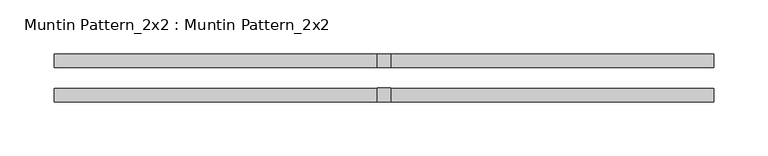
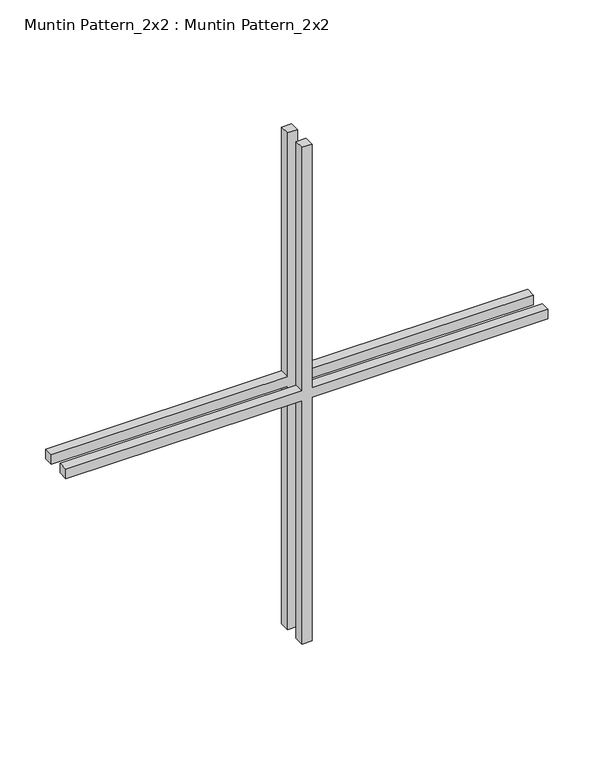
"""IFC4 building model written with IfcOpenShell, lengths in millimetres: proxy geometry, Muntin Pattern_2x2 : Muntin Pattern_2x2."""

from ifc_helpers import new_model, si_unit, frame, origin, place, context, project, spatial, polyline, outline, extrude, source, transform, mapped, element, save


def muntin_pattern_2x2_muntin_pattern_2x2_0ab70a76(model_context):
    return source(origin(), model_context, "Body", "SweptSolid", [
        extrude(outline(polyline([(338.1375, -6.35), (338.1375, -304.8), (325.4375, -304.8), (325.4375, -6.35), (0.0, -6.35), (0.0, 6.35), (325.4375, 6.35), (325.4375, 304.8), (338.1375, 304.8), (338.1375, 6.35), (663.575, 6.35), (663.575, -6.35), (338.1375, -6.35)])), frame((0.0, -22.225, 0.0), z_axis=(0.0, 1.0, 0.0), x_axis=(0.0, 0.0, 1.0)), (0.0, 0.0, 1.0), 12.7),
        extrude(outline(polyline([(338.1375, -6.35), (338.1375, -304.8), (325.4375, -304.8), (325.4375, -6.35), (0.0, -6.35), (0.0, 6.35), (325.4375, 6.35), (325.4375, 304.8), (338.1375, 304.8), (338.1375, 6.35), (663.575, 6.35), (663.575, -6.35), (338.1375, -6.35)])), frame((0.0, 9.525, 0.0), z_axis=(0.0, 1.0, 0.0), x_axis=(0.0, 0.0, 1.0)), (0.0, 0.0, 1.0), 12.7),
    ])


if __name__ == "__main__":
    model = new_model("IFC4")
    model_context = context("Model", 3, world=origin())
    ifc_project = project(units=[si_unit("LENGTHUNIT", "METRE", prefix="MILLI")], contexts=[model_context])
    site = spatial("IfcSite", under=ifc_project)
    building = spatial("IfcBuilding", under=site)
    placement = place(None, origin())
    muntin_pattern_2x2_muntin_pattern_2x2_shape = muntin_pattern_2x2_muntin_pattern_2x2_0ab70a76(model_context)
    element("IfcBuildingElementProxy", 1, Name="Muntin Pattern_2x2 : Muntin Pattern_2x2", ObjectType="Muntin Pattern_2x2 : Muntin Pattern_2x2", at=placement, inside=building, context=model_context, shape_type="MappedRepresentation", body=[
        mapped(muntin_pattern_2x2_muntin_pattern_2x2_shape, transform((0.0, 0.0, 0.0), x_axis=(1.0, 0.0, 0.0), y_axis=(0.0, 1.0, 0.0), z_axis=(0.0, 0.0, 1.0))),
    ])
    save(model, "model.ifc")

# Revit data of these elements
# Type "Muntin Pattern_2x2 : Muntin Pattern_2x2"
#   Width [instance default] = 4' - 0"
#   Thickness = 0' - 0 1/2"
#   Height [instance default] = 4' - 0"
#   Distance = 0' - 0 3/4"
#   Interior Material [instance default] = none
#   Exterior Material [instance default] = none
#   Default Elevation = 0
# Element 1 (IfcBuildingElementProxy, "Muntin Pattern_2x2 : Muntin Pattern_2x2")
#   Width = 2' - 0"
#   Height = 2' - 2 1/8"
#   Interior Material = Wood - Stained
#   Exterior Material = Clad - White
#   Materials on its faces: "Clad - White", "Wood - Stained"
# Materials
#   "Clad - White": class "Wood", colour RGB 242 242 238, transparency 0, Cost = 0
#   "Wood - Stained": class "Wood", colour RGB 224 178 126, transparency 0, Cost = 0
